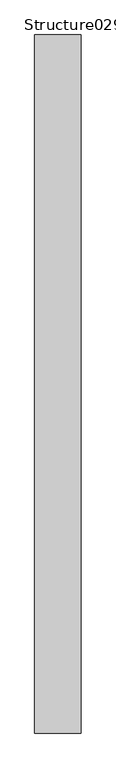
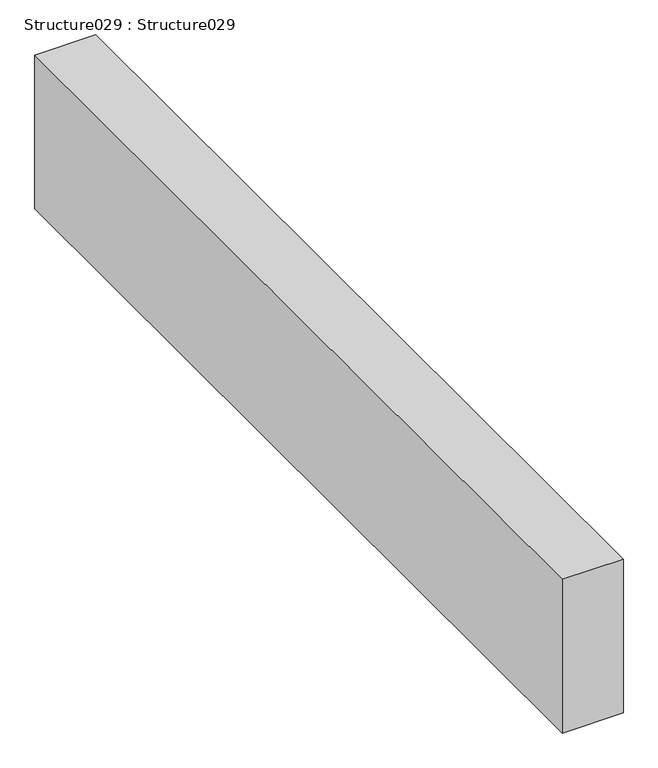
"""IFC4 building model written with IfcOpenShell, lengths in millimetres: proxy geometry, Structure029 : Structure029."""

from ifc_helpers import new_model, si_unit, frame, origin, place, context, project, spatial, polyline, outline, extrude, source, transform, mapped, element, save


def structure029_structure029_cb0ead45(model_context):
    return source(origin(), model_context, "Body", "SweptSolid", [
        extrude(outline(polyline([(-9298.3737014, 7982.1531721), (-9431.7237014, 7982.1531721), (-9431.7237014, 9982.1531721), (-9298.3737014, 9982.1531721), (-9298.3737014, 7982.1531721)])), frame((0.0, 0.0, 39579.2960083), z_axis=(0.0, 0.0, 1.0), x_axis=(1.0, 0.0, 0.0)), (0.0, 0.0, 1.0), 355.6),
    ])


if __name__ == "__main__":
    model = new_model("IFC4")
    model_context = context("Model", 3, world=origin())
    ifc_project = project(units=[si_unit("LENGTHUNIT", "METRE", prefix="MILLI")], contexts=[model_context])
    site = spatial("IfcSite", under=ifc_project)
    building = spatial("IfcBuilding", under=site)
    placement = place(None, origin())
    structure029_structure029_shape = structure029_structure029_cb0ead45(model_context)
    element("IfcBuildingElementProxy", 1, Name="Structure029 : Structure029", ObjectType="Structure029 : Structure029", at=placement, inside=building, context=model_context, shape_type="MappedRepresentation", body=[
        mapped(structure029_structure029_shape, transform((0.0, 0.0, 0.0), x_axis=(1.0, 0.0, 0.0), y_axis=(0.0, 1.0, 0.0), z_axis=(0.0, 0.0, 1.0))),
    ])
    save(model, "model.ifc")

# Revit data of these elements
# Type "Structure029 : Structure029"
#   NameOverride = "Structure029"
# Element 1 (IfcBuildingElementProxy, "Structure029 : Structure029")
#   Materials on its faces: "STRUCTURAL MEMBER (SEE STRUCTURAL DWGS)"
# Materials
#   "STRUCTURAL MEMBER (SEE STRUCTURAL DWGS)": class "Unassigned", colour RGB 176 134 95, transparency 0, Cost = 0
